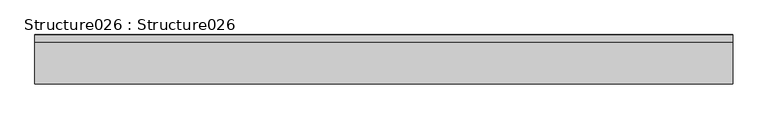
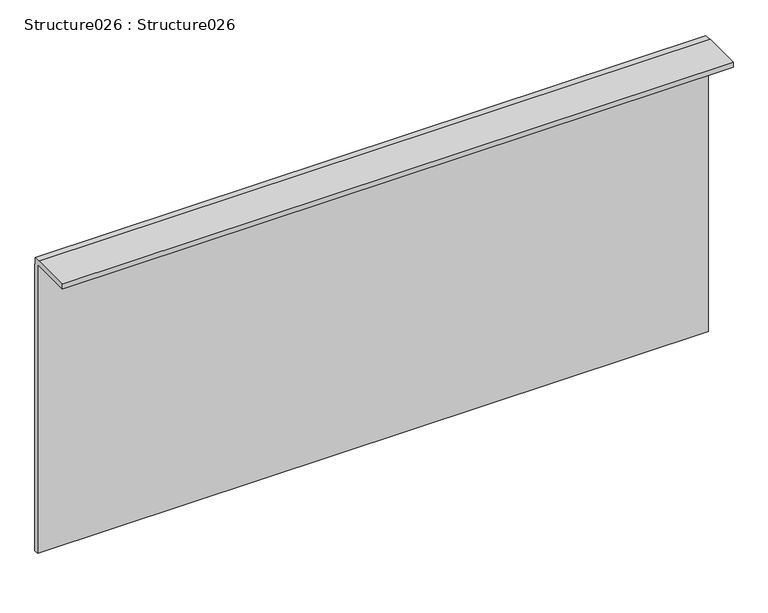
"""IFC4 building model written with IfcOpenShell, lengths in millimetres: proxy geometry, Structure026 : Structure026."""

from ifc_helpers import new_model, si_unit, frame, origin, place, context, project, spatial, polyline, outline, extrude, source, transform, mapped, element, save


def structure026_structure026_8ede5679(model_context):
    return source(origin(), model_context, "Body", "SweptSolid", [
        extrude(outline(polyline([(-4250.1925368, 41062.4264687), (-4377.546792, 41062.4264687), (-4377.546792, 41077.896), (-4258.3374811, 41077.896), (-4258.3374811, 41076.616), (-4237.1842972, 41076.616), (-4237.1842972, 41055.4628161), (-4235.9042972, 41055.4628161), (-4235.9042972, 40150.796), (-4250.1925368, 40150.796), (-4250.1925368, 41062.4264687)])), frame((12382.5, 0.0, 0.0), z_axis=(1.0, 0.0, 0.0), x_axis=(0.0, 1.0, 0.0)), (0.0, 0.0, 1.0), 2000.0),
    ])


if __name__ == "__main__":
    model = new_model("IFC4")
    model_context = context("Model", 3, world=origin())
    ifc_project = project(units=[si_unit("LENGTHUNIT", "METRE", prefix="MILLI")], contexts=[model_context])
    site = spatial("IfcSite", under=ifc_project)
    building = spatial("IfcBuilding", under=site)
    placement = place(None, origin())
    structure026_structure026_shape = structure026_structure026_8ede5679(model_context)
    element("IfcBuildingElementProxy", 1, Name="Structure026 : Structure026", ObjectType="Structure026 : Structure026", at=placement, inside=building, context=model_context, shape_type="MappedRepresentation", body=[
        mapped(structure026_structure026_shape, transform((0.0, 0.0, 0.0), x_axis=(1.0, 0.0, 0.0), y_axis=(0.0, 1.0, 0.0), z_axis=(0.0, 0.0, 1.0))),
    ])
    save(model, "model.ifc")

# Revit data of these elements
# Type "Structure026 : Structure026"
#   NameOverride = "Structure026"
# Element 1 (IfcBuildingElementProxy, "Structure026 : Structure026")
#   Materials on its faces: "5/8\"  GYPSUM BOARD"
# Materials
#   "5/8\"  GYPSUM BOARD": class "Unassigned", colour RGB 255 255 255, transparency 0, Cost = 0
